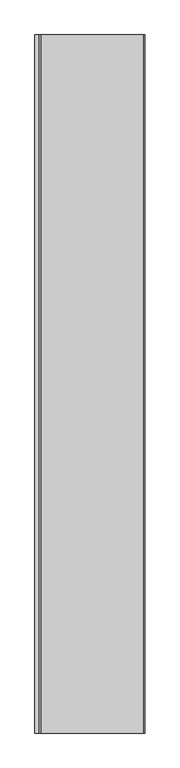
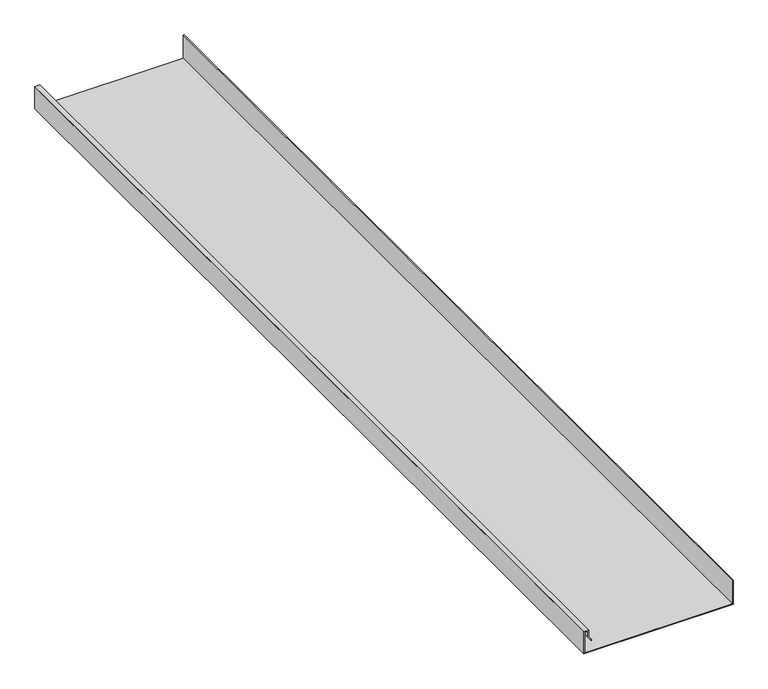
"""IFC4 building model written with IfcOpenShell, lengths in millimetres: proxy geometry, Roof006 17120 : Roof006 17120."""

from ifc_helpers import new_model, si_unit, frame, origin, place, context, project, spatial, polyline, outline, extrude, source, transform, mapped, element, save


def generic_models_3436e616(model_context):
    return source(origin(), model_context, "Body", "SweptSolid", [
        extrude(outline(polyline([(41812.1344716, 5824.6669376), (41802.3258778, 5831.7826603), (41803.5002989, 5833.4015288), (41812.7835259, 5826.6669376), (41827.6196278, 5826.6669376), (41827.6196278, 5815.9921329), (41778.8024403, 5815.9921329), (41778.8024403, 6130.426215), (41832.5758778, 6130.426215), (41832.5758778, 6128.426215), (41780.8024403, 6128.426215), (41780.8024403, 5817.9921329), (41825.6196278, 5817.9921329), (41825.6196278, 5824.6669376), (41812.1344716, 5824.6669376)])), frame((0.0, 2217.3609988, 0.0), z_axis=(0.0, 1.0, 0.0), x_axis=(0.0, 0.0, 1.0)), (0.0, 0.0, 1.0), 2000.0),
    ])


if __name__ == "__main__":
    model = new_model("IFC4")
    model_context = context("Model", 3, world=origin())
    ifc_project = project(units=[si_unit("LENGTHUNIT", "METRE", prefix="MILLI")], contexts=[model_context])
    site = spatial("IfcSite", under=ifc_project)
    building = spatial("IfcBuilding", under=site)
    placement = place(None, origin())
    generic_models_shape = generic_models_3436e616(model_context)
    element("IfcBuildingElementProxy", 1, Name="Roof006 17120 : Roof006 17120", ObjectType="Roof006 17120 : Roof006 17120", at=placement, inside=building, context=model_context, shape_type="MappedRepresentation", body=[
        mapped(generic_models_shape, transform((0.0, 0.0, 0.0), x_axis=(1.0, 0.0, 0.0), y_axis=(0.0, 1.0, 0.0), z_axis=(0.0, 0.0, 1.0))),
    ])
    save(model, "model.ifc")

# Revit data of these elements
# Type "Roof006 17120 : Roof006 17120"
#   NameOverride = "Roof006"
# Element 1 (IfcBuildingElementProxy, "Roof006 17120 : Roof006 17120")
#   Materials on its faces: "STANDING SEAM METAL ROOF FOLLOW MANU. RECOMMENDED EDGE/TRANSITION DETAILS"
# Materials
#   "STANDING SEAM METAL ROOF FOLLOW MANU. RECOMMENDED EDGE/TRANSITION DETAILS": class "Unassigned", colour RGB 128 128 128, transparency 0, Cost = 0
